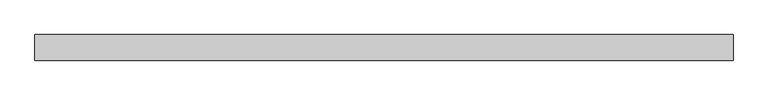
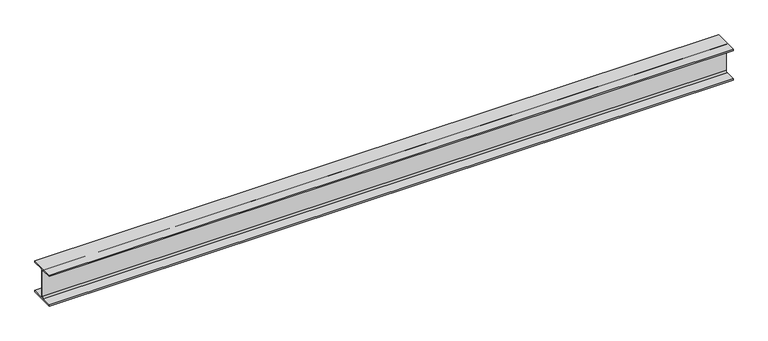
"""IFC4 building model written with IfcOpenShell, lengths in millimetres: beam geometry, 0912_Steel Framing_H-KSD3502 : H_SB_ASB_H-390x300x10x16."""

from ifc_helpers import new_model, si_unit, point, frame, frame_2d, origin, place, context, project, spatial, polyline, circle_curve, trimmed, segment, composite_curve, outline, extrude, source, transform, mapped, element, save


def beam_d2c522c6(model_context):
    return source(origin(), model_context, "Body", "SweptSolid", [
        extrude(outline(composite_curve([segment(polyline([(150.0, -179.0), (150.0, -195.0), (-150.0, -195.0), (-150.0, -179.0), (-27.0, -179.0)]), True, "CONTINUOUS"), segment(trimmed(circle_curve(frame_2d((-27.0, -157.0)), 22.0), [point((-27.0, -179.0))], [point((-5.0, -157.0))], True, "CARTESIAN"), True, "CONTINUOUS"), segment(polyline([(-5.0, -157.0), (-5.0, 157.0)]), True, "CONTINUOUS"), segment(trimmed(circle_curve(frame_2d((-27.0, 157.0)), 22.0), [point((-5.0, 157.0))], [point((-27.0, 179.0))], True, "CARTESIAN"), True, "CONTINUOUS"), segment(polyline([(-27.0, 179.0), (-150.0, 179.0), (-150.0, 195.0), (150.0, 195.0), (150.0, 179.0), (27.0, 179.0)]), True, "CONTINUOUS"), segment(trimmed(circle_curve(frame_2d((27.0, 157.0)), 22.0), [point((27.0, 179.0))], [point((5.0, 157.0))], True, "CARTESIAN"), True, "CONTINUOUS"), segment(polyline([(5.0, 157.0), (5.0, -157.0)]), True, "CONTINUOUS"), segment(trimmed(circle_curve(frame_2d((27.0, -157.0)), 22.0), [point((5.0, -157.0))], [point((27.0, -179.0))], True, "CARTESIAN"), True, "CONTINUOUS"), segment(polyline([(27.0, -179.0), (150.0, -179.0)]), True, "CONTINUOUS")], self_intersect=False)), frame((-4087.3, 0.0, 0.0), z_axis=(1.0, 0.0, 0.0), x_axis=(0.0, 1.0, 0.0)), (0.0, 0.0, 1.0), 8174.6),
    ])


if __name__ == "__main__":
    model = new_model("IFC4")
    model_context = context("Model", 3, world=origin())
    ifc_project = project(units=[si_unit("LENGTHUNIT", "METRE", prefix="MILLI")], contexts=[model_context])
    site = spatial("IfcSite", under=ifc_project)
    building = spatial("IfcBuilding", under=site)
    placement = place(None, origin())
    beam_shape = beam_d2c522c6(model_context)
    element("IfcBeam", 1, ObjectType="0912_Steel Framing_H-KSD3502 : H_SB_ASB_H-390x300x10x16", at=placement, inside=building, context=model_context, shape_type="MappedRepresentation", body=[
        mapped(beam_shape, transform((0.0, 0.0, 0.0), x_axis=(1.0, 0.0, 0.0), y_axis=(0.0, 1.0, 0.0), z_axis=(0.0, 0.0, 1.0))),
    ])
    save(model, "model.ifc")

# Revit data of these elements
# Type "0912_Steel Framing_H-KSD3502 : H_SB_ASB_H-390x300x10x16"
#   H_WM Code_1 = "S01AA001-00001 | Main Steel Structure Fabrication Work | Shelter/Building | Heavy Steel - Standard (Weight≥90KG/M) | Material: (   )"
#   H_WM Code_2 = "S03AA027-00001 | Main Steel Structure Erection Work | Shelter/Building | Heavy Steel (Weight≥90KG/M) | Material: (   )"
#   H_WM Code_3 = "S01AA010-00001 | Main Steel Structure Fabrication Work | Shelter/Building | Steel Painting/Coating | for Non-Fireproofed Steel Surface, Surface Preparation, Primer, Second & Final Coat | Material: (   )"
#   H_Q'ty Cal Type Tag = "SB-Q2"
#   Width = 30.0 cm
#   Web Thickness = 1.0 cm
#   Web Fillet = 2.2 cm
#   Warping Constant = 2520000.0 cm⁶
#   W = 0
#   Torsional Moment of Inertia = 94.3867 cm⁴
#   Section Area = 136.0 cm²
#   Plastic Modulus weak axis = 733.0 cm³
#   Plastic Modulus strong axis = 2190.0 cm³
#   Perimeter = 1.92 m²/m
#   Nominal Weight = 107.00 kgf/m
#   Moment of Inertia weak axis = 7210.00 cm⁴
#   Moment of Inertia strong axis = 38700.00 cm⁴
#   Height = 39.0 cm
#   Flange Thickness = 1.6 cm
#   Elastic Modulus weak axis = 481.0 cm³
#   Elastic Modulus strong axis = 1980.0 cm³
#   Centroid Vertical = 19.5 cm
#   Centroid Horizontal = 15.0 cm
#   Ix = 387000000
#   Length [instance default] = 1.5240 m
#   Zx = 2190000
#   b = 0.3000 m
#   h = 0.3900 m
#   r = 0.0220 m
#   s = 0.0100 m
#   t = 0.0160 m
#   A = 0.0136 m²
#   Structural Material [instance default] = Steel, 45-345
#   Assembly Code = ""
# Element 1 (IfcBeam, "0912_Steel Framing_H-KSD3502 : H_SB_ASB_H-390x300x10x16")
#   Structural Material = none
# Materials
#   "Steel, 45-345": class "Metal", colour RGB 189 187 185, transparency 0, Description = "Steel 345 MPa", Cost = 0
